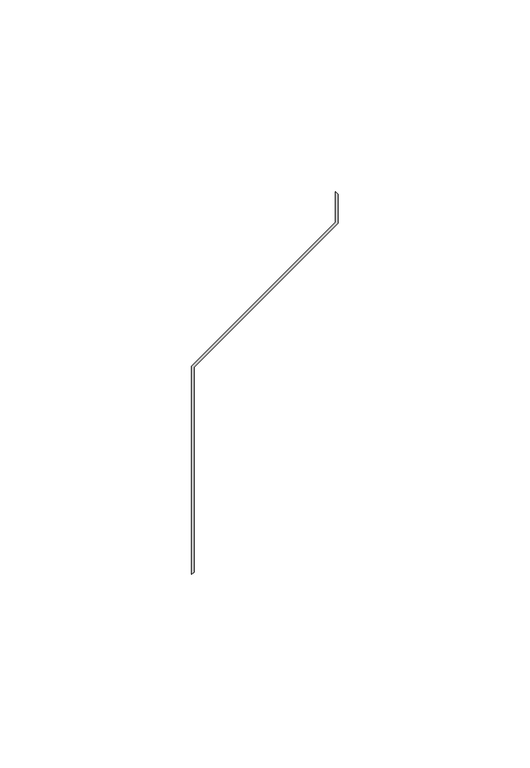
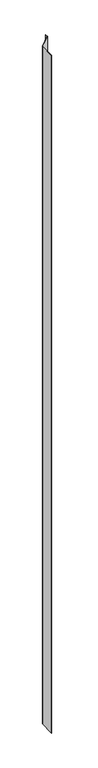
"""IFC4 building model written with IfcOpenShell, lengths in millimetres: proxy geometry, MBCI 7.2-V Panel20 : MBCI 7.2-V Panel-1."""

from ifc_helpers import new_model, si_unit, frame, origin, place, context, project, spatial, polyline, outline, extrude, source, transform, mapped, element, save


def generic_models_939c724f(model_context):
    return source(origin(), model_context, "Body", "SweptSolid", [
        extrude(outline(polyline([(587328.4903864, -534040.6765068), (587328.4903864, -534094.1152716), (587327.8950739, -534094.7105841), (587327.8950739, -534040.4299202), (587365.3854739, -534002.9395202), (587365.3854739, -533995.0663841), (587365.9807864, -533995.6616966), (587365.9807864, -534003.1861068), (587328.4903864, -534040.6765068)])), frame((0.0, 0.0, 12.7), z_axis=(0.0, 0.0, 1.0), x_axis=(1.0, 0.0, 0.0)), (0.0, 0.0, 1.0), 2425.7),
    ])


if __name__ == "__main__":
    model = new_model("IFC4")
    model_context = context("Model", 3, world=origin())
    ifc_project = project(units=[si_unit("LENGTHUNIT", "METRE", prefix="MILLI")], contexts=[model_context])
    site = spatial("IfcSite", under=ifc_project)
    building = spatial("IfcBuilding", under=site)
    placement = place(None, origin())
    generic_models_shape = generic_models_939c724f(model_context)
    element("IfcBuildingElementProxy", 1, Name="MBCI 7.2-V Panel20 : MBCI 7.2-V Panel-1", ObjectType="MBCI 7.2-V Panel20 : MBCI 7.2-V Panel-1", at=placement, inside=building, context=model_context, shape_type="MappedRepresentation", body=[
        mapped(generic_models_shape, transform((0.0, 0.0, 0.0), x_axis=(1.0, 0.0, 0.0), y_axis=(0.0, 1.0, 0.0), z_axis=(0.0, 0.0, 1.0))),
    ])
    save(model, "model.ifc")

# Revit data of these elements
# Element 1 (IfcBuildingElementProxy, "MBCI 7.2-V Panel20 : MBCI 7.2-V Panel-1")
#   Materials on its faces: "MTL PANEL"
# Materials
#   "MTL PANEL": class "Generic", colour RGB 239 242 240, transparency 0, Cost = 0
